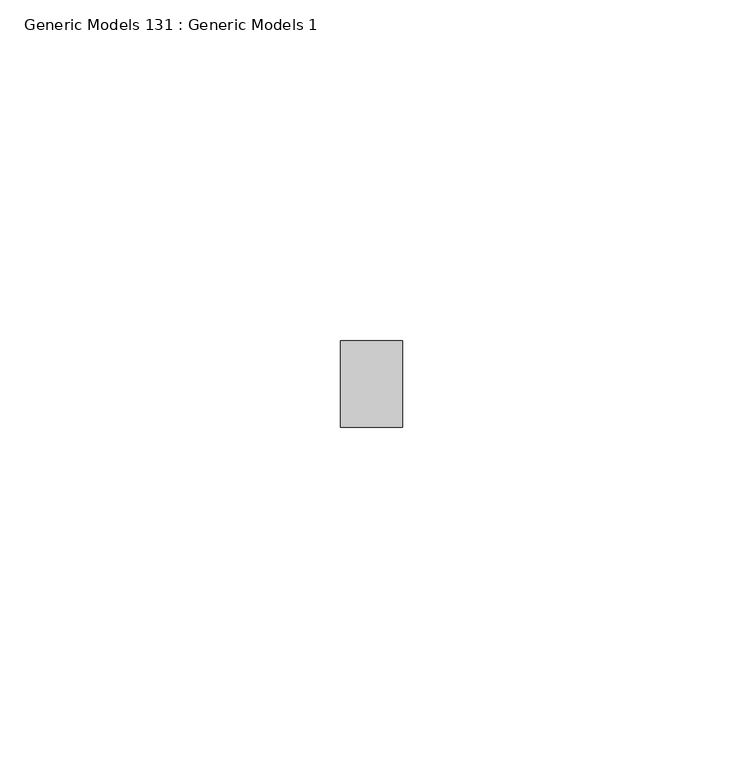
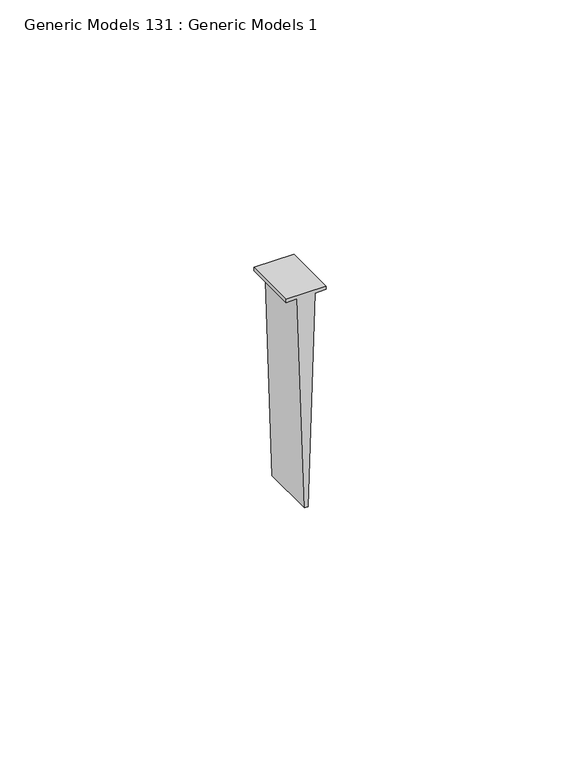
"""IFC4 building model written with IfcOpenShell, lengths in millimetres: proxy geometry, Generic Models 131 : Generic Models 1."""

from ifc_helpers import new_model, si_unit, frame, origin, place, context, project, spatial, polyline, outline, extrude, source, transform, mapped, element, save


def generic_models_131_generic_models_1_0d528cbe(model_context):
    return source(origin(), model_context, "Body", "SweptSolid", [
        extrude(outline(polyline([(-2148.0421376, 49751.7340639), (-2148.8358876, 49751.7340639), (-2148.8358876, 49754.2839275), (-2199.6358876, 49755.8813166), (-2199.6358876, 49756.6800112), (-2148.8358876, 49758.2774003), (-2148.8358876, 49760.8272639), (-2148.0421376, 49760.8272639), (-2148.0421376, 49751.7340639)])), frame((0.0, 565.15, 0.0), z_axis=(0.0, 1.0, 0.0), x_axis=(0.0, 0.0, 1.0)), (0.0, 0.0, 1.0), 12.7),
    ])


if __name__ == "__main__":
    model = new_model("IFC4")
    model_context = context("Model", 3, world=origin())
    ifc_project = project(units=[si_unit("LENGTHUNIT", "METRE", prefix="MILLI")], contexts=[model_context])
    site = spatial("IfcSite", under=ifc_project)
    building = spatial("IfcBuilding", under=site)
    placement = place(None, origin())
    generic_models_131_generic_models_1_shape = generic_models_131_generic_models_1_0d528cbe(model_context)
    element("IfcBuildingElementProxy", 1, Name="Generic Models 131 : Generic Models 1", ObjectType="Generic Models 131 : Generic Models 1", at=placement, inside=building, context=model_context, shape_type="MappedRepresentation", body=[
        mapped(generic_models_131_generic_models_1_shape, transform((0.0, 0.0, 0.0), x_axis=(1.0, 0.0, 0.0), y_axis=(0.0, 1.0, 0.0), z_axis=(0.0, 0.0, 1.0))),
    ])
    save(model, "model.ifc")

# Revit data of these elements
# Element 1 (IfcBuildingElementProxy, "Generic Models 131 : Generic Models 1")
#   Materials on its faces: "METAL RUNNER CHANNEL; FASTEN @ 24\" O.C."
# Materials
#   "METAL RUNNER CHANNEL; FASTEN @ 24\" O.C.": class "Unassigned", colour RGB 210 209 208, transparency 0, Keynote = "M05121300.02", Cost = 0
